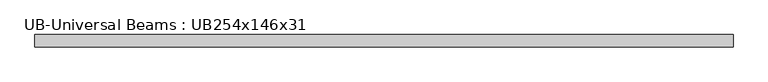
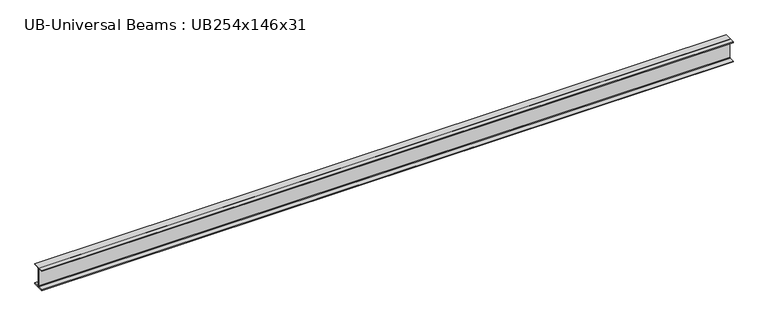
"""IFC4 building model written with IfcOpenShell, lengths in millimetres: beam geometry, UB-Universal Beams : UB254x146x31."""

from ifc_helpers import new_model, si_unit, point, frame, frame_2d, origin, place, context, project, spatial, polyline, circle_curve, trimmed, segment, composite_curve, outline, extrude, source, transform, mapped, element, save


def ub_universal_beams_ub254x146x31_9e4386c4(model_context):
    return source(origin(), model_context, "Body", "SweptSolid", [
        extrude(outline(composite_curve([segment(polyline([(73.05, -117.1), (73.05, -125.7), (-73.05, -125.7), (-73.05, -117.1), (-10.6, -117.1)]), True, "CONTINUOUS"), segment(trimmed(circle_curve(frame_2d((-10.6, -109.5)), 7.6), [point((-10.6, -117.1))], [point((-3.0, -109.5))], True, "CARTESIAN"), True, "CONTINUOUS"), segment(polyline([(-3.0, -109.5), (-3.0, 109.5)]), True, "CONTINUOUS"), segment(trimmed(circle_curve(frame_2d((-10.6, 109.5)), 7.6), [point((-3.0, 109.5))], [point((-10.6, 117.1))], True, "CARTESIAN"), True, "CONTINUOUS"), segment(polyline([(-10.6, 117.1), (-73.05, 117.1), (-73.05, 125.7), (73.05, 125.7), (73.05, 117.1), (10.6, 117.1)]), True, "CONTINUOUS"), segment(trimmed(circle_curve(frame_2d((10.6, 109.5)), 7.6), [point((10.6, 117.1))], [point((3.0, 109.5))], True, "CARTESIAN"), True, "CONTINUOUS"), segment(polyline([(3.0, 109.5), (3.0, -109.5)]), True, "CONTINUOUS"), segment(trimmed(circle_curve(frame_2d((10.6, -109.5)), 7.6), [point((3.0, -109.5))], [point((10.6, -117.1))], True, "CARTESIAN"), True, "CONTINUOUS"), segment(polyline([(10.6, -117.1), (73.05, -117.1)]), True, "CONTINUOUS")], self_intersect=False)), frame((-4141.1, 0.0, 0.0), z_axis=(1.0, 0.0, 0.0), x_axis=(0.0, 1.0, 0.0)), (0.0, 0.0, 1.0), 8282.2),
    ])


if __name__ == "__main__":
    model = new_model("IFC4")
    model_context = context("Model", 3, world=origin())
    ifc_project = project(units=[si_unit("LENGTHUNIT", "METRE", prefix="MILLI")], contexts=[model_context])
    site = spatial("IfcSite", under=ifc_project)
    building = spatial("IfcBuilding", under=site)
    placement = place(None, origin())
    ub_universal_beams_ub254x146x31_shape = ub_universal_beams_ub254x146x31_9e4386c4(model_context)
    element("IfcBeam", 1, ObjectType="UB-Universal Beams : UB254x146x31", at=placement, inside=building, context=model_context, shape_type="MappedRepresentation", body=[
        mapped(ub_universal_beams_ub254x146x31_shape, transform((0.0, 0.0, 0.0), x_axis=(1.0, 0.0, 0.0), y_axis=(0.0, 1.0, 0.0), z_axis=(0.0, 0.0, 1.0))),
    ])
    save(model, "model.ifc")

# Revit data of these elements
# Type "UB-Universal Beams : UB254x146x31"
#   Section Name Key = "UB254X146X31"
#   Width = 14.61 cm
#   Web Thickness = 0.6 cm
#   Web Fillet = 0.76 cm
#   Warping Constant = 66000.0 cm⁶
#   Torsional Moment of Inertia = 8.55 cm⁴
#   Section Area = 39.7 cm²
#   Plastic Modulus weak axis = 94.1 cm³
#   Plastic Modulus strong axis = 393.0 cm³
#   Nominal Weight = 31.10 kgf/m
#   Moment of Inertia weak axis = 448.00 cm⁴
#   Moment of Inertia strong axis = 4413.00 cm⁴
#   Height = 25.14 cm
#   Flange Thickness = 0.86 cm
#   Elastic Modulus weak axis = 61.3 cm³
#   Elastic Modulus strong axis = 351.0 cm³
#   Centroid Vertical = 12.57 cm
#   Centroid Horizontal = 7.305 cm
#   Bolt Spacing = 7.0 cm
#   Length [instance default] = 1500 mm
#   Structural Material [instance default] = Metal - Steel 43-275
#   Type Comments = ""
#   Assembly Code = ""
# Element 1 (IfcBeam, "UB-Universal Beams : UB254x146x31")
#   Materials on its faces: "Metal - Steel 43-275"
# Materials
#   "Metal - Steel 43-275": class "Metal", colour RGB 247 247 247, transparency 0, Cost = 0
